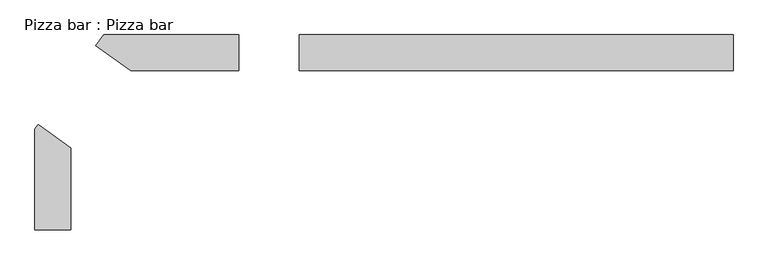
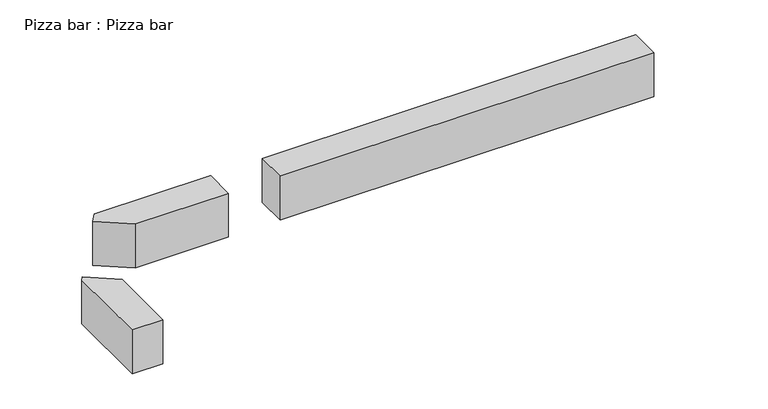
"""IFC4 building model written with IfcOpenShell, lengths in millimetres: furniture geometry, Pizza bar : Pizza bar."""

from ifc_helpers import new_model, si_unit, origin, origin_with_axes, place, context, project, spatial, polyline, outline, extrude, source, transform, mapped, element, save


def pizza_bar_pizza_bar_91474dbc(model_context):
    return source(origin(), model_context, "Body", "SweptSolid", [
        extrude(outline(polyline([(-54731.6752252, 253412.373516), (-54731.6752252, 255698.6421926), (-54656.3205969, 255802.3589406), (-53918.8752252, 255266.573516), (-53918.8752252, 253412.373516), (-54731.6752252, 253412.373516)])), origin_with_axes(), (0.0, 0.0, 1.0), 1219.2),
        extrude(outline(polyline([(-53177.4958112, 257830.2096813), (-50119.529344, 257830.2096813), (-50119.529344, 257017.4096813), (-52567.1277344, 257017.4096813), (-53353.1281953, 257588.4724432), (-53177.4958112, 257830.2096813)])), origin_with_axes(), (0.0, 0.0, 1.0), 1219.2),
        extrude(outline(polyline([(-38945.0551606, 257830.2096813), (-38945.0551606, 257017.4096813), (-48756.3723171, 257017.4096813), (-48756.3723171, 257830.2096813), (-38945.0551606, 257830.2096813)])), origin_with_axes(), (0.0, 0.0, 1.0), 1219.2),
    ])


if __name__ == "__main__":
    model = new_model("IFC4")
    model_context = context("Model", 3, world=origin())
    ifc_project = project(units=[si_unit("LENGTHUNIT", "METRE", prefix="MILLI")], contexts=[model_context])
    site = spatial("IfcSite", under=ifc_project)
    building = spatial("IfcBuilding", under=site)
    placement = place(None, origin())
    pizza_bar_pizza_bar_shape = pizza_bar_pizza_bar_91474dbc(model_context)
    element("IfcFurniture", 1, ObjectType="Pizza bar : Pizza bar", at=placement, inside=building, context=model_context, shape_type="MappedRepresentation", body=[
        mapped(pizza_bar_pizza_bar_shape, transform((0.0, 0.0, 0.0), x_axis=(1.0, 0.0, 0.0), y_axis=(0.0, 1.0, 0.0), z_axis=(0.0, 0.0, 1.0))),
    ])
    save(model, "model.ifc")

# Revit data of these elements
# Element 1 (IfcFurniture, "Pizza bar : Pizza bar")
#   Materials on its faces: "PIZZA BAR"
# Materials
#   "PIZZA BAR": class "Generic", colour RGB 187 187 187, transparency 0, Cost = 0
